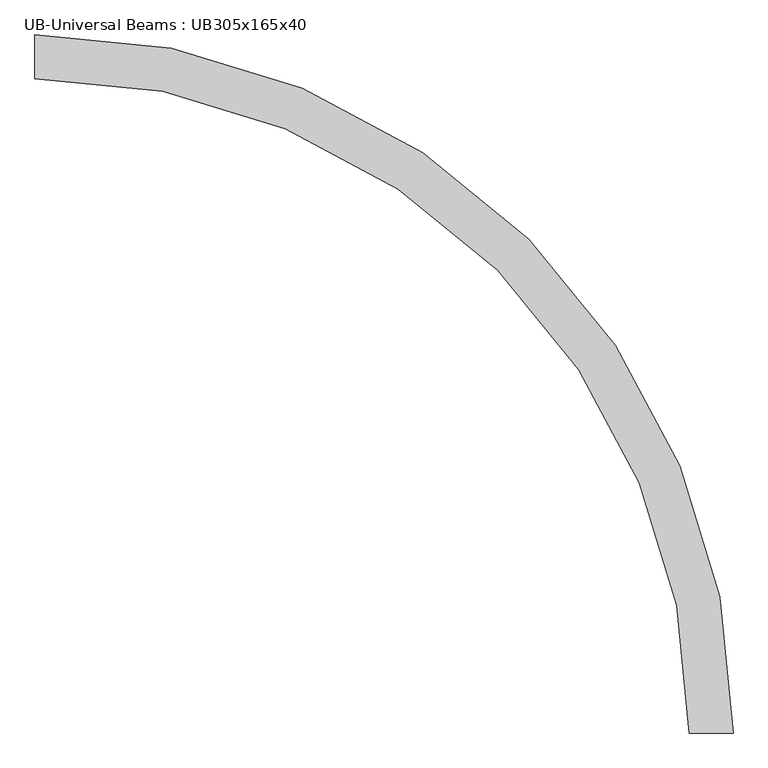
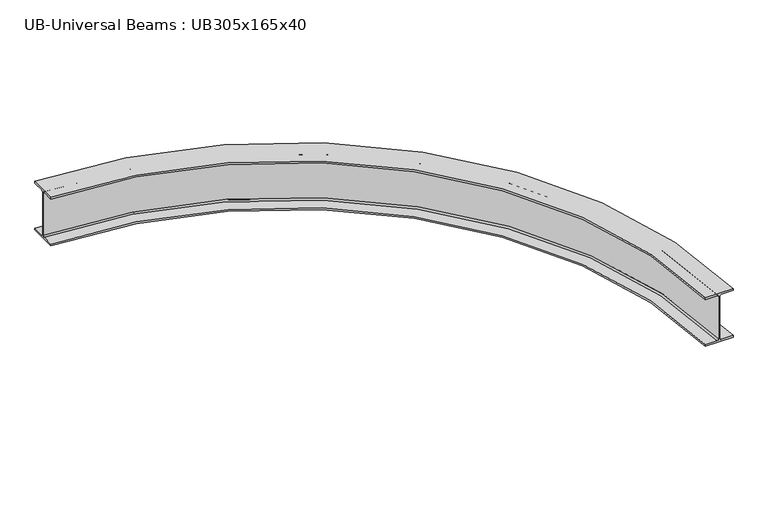
"""IFC4 building model written with IfcOpenShell, lengths in millimetres: beam geometry, UB-Universal Beams : UB305x165x40."""

from ifc_helpers import new_model, si_unit, point, frame, origin, place, context, project, spatial, polyline, circle_curve, ellipse_curve, trimmed, source, transform, mapped, element, save
from ifc_brep_helpers import plane_surface, cylinder_surface, revolved_surface, advanced_brep


def ub_universal_beams_ub305x165x40_ea4b1fef(model_context):
    return source(origin(), model_context, "Body", "AdvancedBrep", [
        advanced_brep(
        [(2628.0844123, -2545.5844123, -141.5), (2557.4844123, -2545.5844123, -141.5), (2548.5844123, -2545.5844123, -132.6), (2548.5844123, -2545.5844123, 132.6), (2557.4844123, -2545.5844123, 141.5), (2628.0844123, -2545.5844123, 141.5), (2628.0844123, -2545.5844123, 151.7), (2463.0844123, -2545.5844123, 151.7), (2463.0844123, -2545.5844123, 141.5), (2533.6844123, -2545.5844123, 141.5), (2542.5844123, -2545.5844123, 132.6), (2542.5844123, -2545.5844123, -132.6), (2533.6844123, -2545.5844123, -141.5), (2463.0844123, -2545.5844123, -141.5), (2463.0844123, -2545.5844123, -151.7), (2628.0844123, -2545.5844123, -151.7), (0.0, 82.5, -141.5), (0.0, 82.5, -151.7), (0.0, -82.5, -151.7), (0.0, -82.5, -141.5), (0.0, -11.9, -141.5), (0.0, -3.0, -132.6), (0.0, -3.0, 132.6), (0.0, -11.9, 141.5), (0.0, -82.5, 141.5), (0.0, -82.5, 151.7), (0.0, 82.5, 151.7), (0.0, 82.5, 141.5), (0.0, 11.9, 141.5), (0.0, 3.0, 132.6), (0.0, 3.0, -132.6), (0.0, 11.9, -141.5)],
        [
            (0, 1),
            (1, 2, circle_curve(frame((2557.4844123, -2545.5844123, -132.6), z_axis=(0.0, 1.0, 0.0), x_axis=(-1.0, 0.0, 0.0)), 8.9)),
            (2, 3),
            (3, 4, circle_curve(frame((2557.4844123, -2545.5844123, 132.6), z_axis=(0.0, 1.0, 0.0), x_axis=(-1.0, 0.0, 0.0)), 8.9)),
            (4, 5),
            (5, 6),
            (6, 7),
            (7, 8),
            (8, 9),
            (9, 10, circle_curve(frame((2533.6844123, -2545.5844123, 132.6), z_axis=(0.0, 1.0, 0.0), x_axis=(-1.0, 0.0, 0.0)), 8.9)),
            (10, 11),
            (11, 12, circle_curve(frame((2533.6844123, -2545.5844123, -132.6), z_axis=(0.0, 1.0, 0.0), x_axis=(-1.0, 0.0, 0.0)), 8.9)),
            (12, 13),
            (13, 14),
            (14, 15),
            (15, 0),
            (16, 17),
            (17, 18),
            (18, 19),
            (19, 20),
            (20, 21, circle_curve(frame((0.0, -11.9, -132.6), z_axis=(1.0, 0.0, 0.0), x_axis=(0.0, -1.0, 0.0)), 8.9)),
            (21, 22),
            (22, 23, circle_curve(frame((0.0, -11.9, 132.6), z_axis=(1.0, 0.0, 0.0), x_axis=(0.0, -1.0, 0.0)), 8.9)),
            (23, 24),
            (24, 25),
            (25, 26),
            (26, 27),
            (27, 28),
            (28, 29, circle_curve(frame((0.0, 11.9, 132.6), z_axis=(1.0, 0.0, 0.0), x_axis=(0.0, -1.0, 0.0)), 8.9)),
            (29, 30),
            (30, 31, circle_curve(frame((0.0, 11.9, -132.6), z_axis=(1.0, 0.0, 0.0), x_axis=(0.0, -1.0, 0.0)), 8.9)),
            (31, 16),
            (0, 16, circle_curve(frame((0.0, -2545.5844123, -141.5), z_axis=(0.0, 0.0, 1.0), x_axis=(0.0, 1.0, 0.0)), 2628.0844123)),
            (31, 1, circle_curve(frame((0.0, -2545.5844123, -141.5), z_axis=(0.0, 0.0, -1.0), x_axis=(0.0, 1.0, 0.0)), 2557.4844123)),
            (30, 2, circle_curve(frame((0.0, -2545.5844123, -132.6), z_axis=(0.0, 0.0, -1.0), x_axis=(0.0, 1.0, 0.0)), 2548.5844123)),
            (29, 3, circle_curve(frame((0.0, -2545.5844123, 132.6), z_axis=(0.0, 0.0, -1.0), x_axis=(0.0, 1.0, 0.0)), 2548.5844123)),
            (28, 4, circle_curve(frame((0.0, -2545.5844123, 141.5), z_axis=(0.0, 0.0, -1.0), x_axis=(0.0, 1.0, 0.0)), 2557.4844123)),
            (27, 5, circle_curve(frame((0.0, -2545.5844123, 141.5), z_axis=(0.0, 0.0, -1.0), x_axis=(0.0, 1.0, 0.0)), 2628.0844123)),
            (26, 6, circle_curve(frame((0.0, -2545.5844123, 151.7), z_axis=(0.0, 0.0, -1.0), x_axis=(0.0, 1.0, 0.0)), 2628.0844123)),
            (25, 7, circle_curve(frame((0.0, -2545.5844123, 151.7), z_axis=(0.0, 0.0, -1.0), x_axis=(0.0, 1.0, 0.0)), 2463.0844123)),
            (24, 8, circle_curve(frame((0.0, -2545.5844123, 141.5), z_axis=(0.0, 0.0, -1.0), x_axis=(0.0, 1.0, 0.0)), 2463.0844123)),
            (23, 9, circle_curve(frame((0.0, -2545.5844123, 141.5), z_axis=(0.0, 0.0, -1.0), x_axis=(0.0, 1.0, 0.0)), 2533.6844123)),
            (22, 10, circle_curve(frame((0.0, -2545.5844123, 132.6), z_axis=(0.0, 0.0, -1.0), x_axis=(0.0, 1.0, 0.0)), 2542.5844123)),
            (21, 11, circle_curve(frame((0.0, -2545.5844123, -132.6), z_axis=(0.0, 0.0, -1.0), x_axis=(0.0, 1.0, 0.0)), 2542.5844123)),
            (20, 12, circle_curve(frame((0.0, -2545.5844123, -141.5), z_axis=(0.0, 0.0, -1.0), x_axis=(0.0, 1.0, 0.0)), 2533.6844123)),
            (19, 13, circle_curve(frame((0.0, -2545.5844123, -141.5), z_axis=(0.0, 0.0, -1.0), x_axis=(0.0, 1.0, 0.0)), 2463.0844123)),
            (18, 14, circle_curve(frame((0.0, -2545.5844123, -151.7), z_axis=(0.0, 0.0, -1.0), x_axis=(0.0, 1.0, 0.0)), 2463.0844123)),
            (17, 15, circle_curve(frame((0.0, -2545.5844123, -151.7), z_axis=(0.0, 0.0, -1.0), x_axis=(0.0, 1.0, 0.0)), 2628.0844123)),
        ],
        [
            plane_surface(frame((2545.5844123, -2545.5844123, 0.0), z_axis=(0.0, -1.0, 0.0), x_axis=(0.0, 0.0, 1.0))),
            plane_surface(frame((0.0, 0.0, 0.0), z_axis=(-1.0, 0.0, 0.0), x_axis=(0.0, 0.0, 1.0))),
            plane_surface(frame((0.0, -2545.5844123, -141.5), z_axis=(0.0, 0.0, 1.0), x_axis=(0.0, 1.0, 0.0))),
            revolved_surface(trimmed(ellipse_curve(frame((0.0, 11.9, -132.6), z_axis=(1.0, 0.0, 0.0), x_axis=(0.0, -1.0, 0.0)), 8.9, 8.9), [point((0.0, 3.0, -132.6))], [point((0.0, 11.9, -141.5))], True, "CARTESIAN"), (0.0, -2545.5844123, 0.0), (0.0, 0.0, -1.0)),
            cylinder_surface(frame((0.0, -2545.5844123, 0.0), z_axis=(0.0, 0.0, -1.0), x_axis=(0.0, 1.0, 0.0)), 2548.5844123),
            revolved_surface(trimmed(ellipse_curve(frame((0.0, 11.9, 132.6), z_axis=(1.0, 0.0, 0.0), x_axis=(0.0, -1.0, 0.0)), 8.9, 8.9), [point((0.0, 11.9, 141.5))], [point((0.0, 3.0, 132.6))], True, "CARTESIAN"), (0.0, -2545.5844123, 0.0), (0.0, 0.0, -1.0)),
            plane_surface(frame((0.0, -2545.5844123, 141.5), z_axis=(0.0, 0.0, -1.0), x_axis=(0.0, 1.0, 0.0))),
            cylinder_surface(frame((0.0, -2545.5844123, 0.0), z_axis=(0.0, 0.0, -1.0), x_axis=(0.0, 1.0, 0.0)), 2628.0844123),
            plane_surface(frame((0.0, -2545.5844123, 151.7), z_axis=(0.0, 0.0, 1.0), x_axis=(0.0, 1.0, 0.0))),
            revolved_surface(polyline([(0.0, -82.5, 141.5), (0.0, -82.5, 151.7)]), (0.0, -2545.5844123, 0.0), (0.0, 0.0, -1.0)),
            revolved_surface(trimmed(ellipse_curve(frame((0.0, -11.9, 132.6), z_axis=(1.0, 0.0, 0.0), x_axis=(0.0, -1.0, 0.0)), 8.9, 8.9), [point((0.0, -3.0, 132.6))], [point((0.0, -11.9, 141.5))], True, "CARTESIAN"), (0.0, -2545.5844123, 0.0), (0.0, 0.0, -1.0)),
            revolved_surface(polyline([(0.0, -3.0, -132.6), (0.0, -3.0, 132.6)]), (0.0, -2545.5844123, 0.0), (0.0, 0.0, -1.0)),
            revolved_surface(trimmed(ellipse_curve(frame((0.0, -11.9, -132.6), z_axis=(1.0, 0.0, 0.0), x_axis=(0.0, -1.0, 0.0)), 8.9, 8.9), [point((0.0, -11.9, -141.5))], [point((0.0, -3.0, -132.6))], True, "CARTESIAN"), (0.0, -2545.5844123, 0.0), (0.0, 0.0, -1.0)),
            revolved_surface(polyline([(0.0, -82.5, -151.7), (0.0, -82.5, -141.5)]), (0.0, -2545.5844123, 0.0), (0.0, 0.0, -1.0)),
            plane_surface(frame((0.0, -2545.5844123, -151.7), z_axis=(0.0, 0.0, -1.0), x_axis=(0.0, 1.0, 0.0))),
        ],
        [
            (0, [[1, 2, 3, 4, 5, 6, 7, 8, 9, 10, 11, 12, 13, 14, 15, 16]]),
            (1, [[17, 18, 19, 20, 21, 22, 23, 24, 25, 26, 27, 28, 29, 30, 31, 32]]),
            (2, [[-1, 33, -32, 34]]),
            (3, [[-2, -34, -31, 35]]),
            (4, [[-3, -35, -30, 36]]),
            (5, [[-4, -36, -29, 37]]),
            (6, [[-5, -37, -28, 38]]),
            (7, [[-6, -38, -27, 39]]),
            (8, [[-7, -39, -26, 40]]),
            (9, [[-8, -40, -25, 41]]),
            (6, [[-9, -41, -24, 42]]),
            (10, [[-10, -42, -23, 43]]),
            (11, [[-11, -43, -22, 44]]),
            (12, [[-12, -44, -21, 45]]),
            (2, [[-13, -45, -20, 46]]),
            (13, [[-14, -46, -19, 47]]),
            (14, [[-15, -47, -18, 48]]),
            (7, [[-16, -48, -17, -33]]),
        ],
    ),
    ])


if __name__ == "__main__":
    model = new_model("IFC4")
    model_context = context("Model", 3, world=origin())
    ifc_project = project(units=[si_unit("LENGTHUNIT", "METRE", prefix="MILLI")], contexts=[model_context])
    site = spatial("IfcSite", under=ifc_project)
    building = spatial("IfcBuilding", under=site)
    placement = place(None, origin())
    ub_universal_beams_ub305x165x40_shape = ub_universal_beams_ub305x165x40_ea4b1fef(model_context)
    element("IfcBeam", 1, ObjectType="UB-Universal Beams : UB305x165x40", at=placement, inside=building, context=model_context, shape_type="MappedRepresentation", body=[
        mapped(ub_universal_beams_ub305x165x40_shape, transform((0.0, 0.0, 0.0), x_axis=(1.0, 0.0, 0.0), y_axis=(0.0, 1.0, 0.0), z_axis=(0.0, 0.0, 1.0))),
    ])
    save(model, "model.ifc")

# Revit data of these elements
# Type "UB-Universal Beams : UB305x165x40"
#   Section Name Key = "UB305X165X40"
#   Width = 16.5 cm
#   Web Thickness = 0.6 cm
#   Web Fillet = 0.89 cm
#   Warping Constant = 164000.0 cm⁶
#   Torsional Moment of Inertia = 14.70 cm⁴
#   Section Area = 51.3 cm²
#   Plastic Modulus weak axis = 142.0 cm³
#   Plastic Modulus strong axis = 623.0 cm³
#   Nominal Weight = 40.2999 kgf/m
#   Moment of Inertia weak axis = 764.00 cm⁴
#   Moment of Inertia strong axis = 8503.00 cm⁴
#   Height = 30.34 cm
#   Flange Thickness = 1.02 cm
#   Elastic Modulus weak axis = 92.6 cm³
#   Elastic Modulus strong axis = 560.0 cm³
#   Centroid Vertical = 15.17 cm
#   Centroid Horizontal = 8.25 cm
#   Bolt Spacing = 9.0 cm
#   Length [instance default] = 1500 mm
#   Structural Material [instance default] = Metal - Steel 43-275
#   Type Comments = ""
#   Assembly Code = ""
# Element 1 (IfcBeam, "UB-Universal Beams : UB305x165x40")
#   Materials on its faces: "Metal - Steel 43-275"
# Materials
#   "Metal - Steel 43-275": class "Metal", colour RGB 247 247 247, transparency 0, Cost = 0
